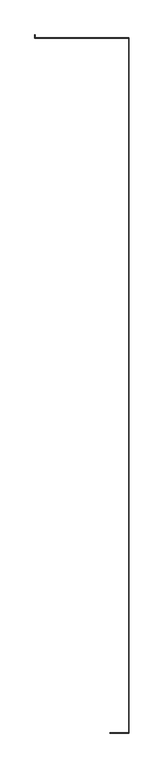
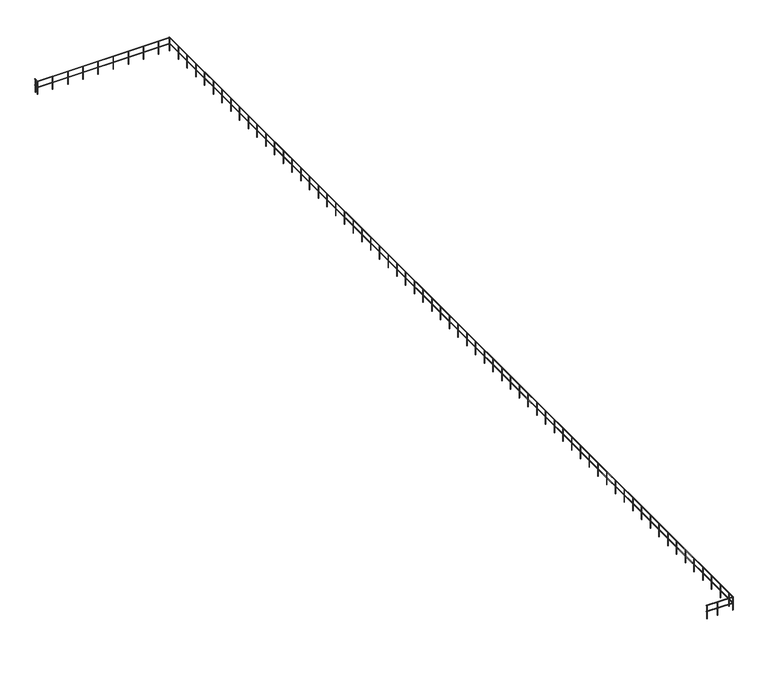
"""IFC4 building model written with IfcOpenShell, lengths in millimetres: railing geometry."""

from ifc_helpers import new_model, si_unit, point, frame, frame_2d, origin, place, context, project, spatial, circle_curve, ellipse_curve, trimmed, segment, composite_curve, outline, extrude, source, transform, mapped, element, save
from ifc_brep_helpers import plane_surface, cylinder_surface, advanced_brep


def railing_6406d98e(model_context):
    return source(origin(), model_context, "Body", "SolidModel", [
        advanced_brep(
        [(65806.3017909, 71787.4208589, 885.0), (65776.3017909, 71787.4208589, 885.0), (65806.3017909, 71467.0208589, 885.0), (65776.3017909, 71437.0208589, 885.0), (76281.0, 71467.0208589, 885.0), (76251.0, 71437.0208589, 885.0), (76281.0, -5867.9791411, 885.0), (76251.0, -5837.9791411, 885.0), (74181.0, -5867.9791411, 885.0), (74181.0, -5837.9791411, 885.0)],
        [
            (0, 1, circle_curve(frame((65791.3017909, 71787.4208589, 885.0), z_axis=(0.0, 1.0, 0.0), x_axis=(-1.0, 0.0, 0.0)), 15.0)),
            (1, 0, circle_curve(frame((65791.3017909, 71787.4208589, 885.0), z_axis=(0.0, 1.0, 0.0), x_axis=(-1.0, 0.0, 0.0)), 15.0)),
            (0, 2),
            (2, 3, ellipse_curve(frame((65791.3017909, 71452.0208589, 885.0), z_axis=(-0.7071067811865464, 0.7071067811865487, 0.0), x_axis=(0.7071067811865487, 0.7071067811865464, 0.0)), 21.2132034, 15.0)),
            (3, 1),
            (3, 2, ellipse_curve(frame((65791.3017909, 71452.0208589, 885.0), z_axis=(-0.7071067811865464, 0.7071067811865487, 0.0), x_axis=(0.7071067811865487, 0.7071067811865464, 0.0)), 21.2132034, 15.0)),
            (2, 4),
            (4, 5, ellipse_curve(frame((76266.0, 71452.0208589, 885.0), z_axis=(-0.7071067811865458, 0.7071067811865492, 0.0), x_axis=(-0.7071067811865492, -0.7071067811865458, 0.0)), 21.2132034, 15.0)),
            (5, 3),
            (5, 4, ellipse_curve(frame((76266.0, 71452.0208589, 885.0), z_axis=(-0.7071067811865458, 0.7071067811865492, 0.0), x_axis=(-0.7071067811865492, -0.7071067811865458, 0.0)), 21.2132034, 15.0)),
            (4, 6),
            (6, 7, ellipse_curve(frame((76266.0, -5852.9791411, 885.0), z_axis=(0.7071067811865491, 0.7071067811865458, 0.0), x_axis=(-0.7071067811865457, 0.7071067811865493, 0.0)), 21.2132034, 15.0)),
            (7, 5),
            (7, 6, ellipse_curve(frame((76266.0, -5852.9791411, 885.0), z_axis=(0.7071067811865491, 0.7071067811865458, 0.0), x_axis=(-0.7071067811865457, 0.7071067811865493, 0.0)), 21.2132034, 15.0)),
            (8, 9, circle_curve(frame((74181.0, -5852.9791411, 885.0), z_axis=(-1.0, 0.0, 0.0), x_axis=(0.0, 1.0, 0.0)), 15.0)),
            (9, 8, circle_curve(frame((74181.0, -5852.9791411, 885.0), z_axis=(-1.0, 0.0, 0.0), x_axis=(0.0, 1.0, 0.0)), 15.0)),
            (6, 8),
            (9, 7),
        ],
        [
            plane_surface(frame((65791.3017909, 71787.4208589, 900.0), z_axis=(0.0, 1.0, 0.0), x_axis=(0.0, 0.0, -1.0))),
            cylinder_surface(frame((65791.3017909, 71787.4208589, 885.0), z_axis=(0.0, 1.0, 0.0), x_axis=(-1.0, 0.0, 0.0)), 15.0),
            cylinder_surface(frame((65791.3017909, 71452.0208589, 885.0), z_axis=(-1.0, 0.0, 0.0), x_axis=(0.0, -1.0, 0.0)), 15.0),
            cylinder_surface(frame((76266.0, 71452.0208589, 885.0), z_axis=(0.0, 1.0, 0.0), x_axis=(-1.0, 0.0, 0.0)), 15.0),
            plane_surface(frame((74181.0, -5852.9791411, 900.0), z_axis=(-1.0, 0.0, 0.0), x_axis=(0.0, -1.0, 0.0))),
            cylinder_surface(frame((76266.0, -5852.9791411, 885.0), z_axis=(1.0, 0.0, 0.0), x_axis=(0.0, 1.0, 0.0)), 15.0),
        ],
        [
            (0, [[1, 2]]),
            (1, [[-1, 3, 4, 5]]),
            (1, [[-2, -5, 6, -3]]),
            (2, [[-4, 7, 8, 9]]),
            (2, [[-6, -9, 10, -7]]),
            (3, [[-8, 11, 12, 13]]),
            (3, [[-10, -13, 14, -11]]),
            (4, [[15, 16]]),
            (5, [[-12, 17, -16, 18]]),
            (5, [[-14, -18, -15, -17]]),
        ],
    ),
        advanced_brep(
        [(65806.3017909, 71787.4208589, 1385.0), (65776.3017909, 71787.4208589, 1385.0), (65806.3017909, 71467.0208589, 1385.0), (65776.3017909, 71437.0208589, 1385.0), (76281.0, 71467.0208589, 1385.0), (76251.0, 71437.0208589, 1385.0), (76281.0, -5867.9791411, 1385.0), (76251.0, -5837.9791411, 1385.0), (74181.0, -5867.9791411, 1385.0), (74181.0, -5837.9791411, 1385.0)],
        [
            (0, 1, circle_curve(frame((65791.3017909, 71787.4208589, 1385.0), z_axis=(0.0, 1.0, 0.0), x_axis=(-1.0, 0.0, 0.0)), 15.0)),
            (1, 0, circle_curve(frame((65791.3017909, 71787.4208589, 1385.0), z_axis=(0.0, 1.0, 0.0), x_axis=(-1.0, 0.0, 0.0)), 15.0)),
            (0, 2),
            (2, 3, ellipse_curve(frame((65791.3017909, 71452.0208589, 1385.0), z_axis=(-0.7071067811865464, 0.7071067811865487, 0.0), x_axis=(0.7071067811865487, 0.7071067811865464, 0.0)), 21.2132034, 15.0)),
            (3, 1),
            (3, 2, ellipse_curve(frame((65791.3017909, 71452.0208589, 1385.0), z_axis=(-0.7071067811865464, 0.7071067811865487, 0.0), x_axis=(0.7071067811865487, 0.7071067811865464, 0.0)), 21.2132034, 15.0)),
            (2, 4),
            (4, 5, ellipse_curve(frame((76266.0, 71452.0208589, 1385.0), z_axis=(-0.7071067811865458, 0.7071067811865492, 0.0), x_axis=(-0.7071067811865492, -0.7071067811865458, 0.0)), 21.2132034, 15.0)),
            (5, 3),
            (5, 4, ellipse_curve(frame((76266.0, 71452.0208589, 1385.0), z_axis=(-0.7071067811865458, 0.7071067811865492, 0.0), x_axis=(-0.7071067811865492, -0.7071067811865458, 0.0)), 21.2132034, 15.0)),
            (4, 6),
            (6, 7, ellipse_curve(frame((76266.0, -5852.9791411, 1385.0), z_axis=(0.7071067811865491, 0.7071067811865458, 0.0), x_axis=(-0.7071067811865457, 0.7071067811865493, 0.0)), 21.2132034, 15.0)),
            (7, 5),
            (7, 6, ellipse_curve(frame((76266.0, -5852.9791411, 1385.0), z_axis=(0.7071067811865491, 0.7071067811865458, 0.0), x_axis=(-0.7071067811865457, 0.7071067811865493, 0.0)), 21.2132034, 15.0)),
            (8, 9, circle_curve(frame((74181.0, -5852.9791411, 1385.0), z_axis=(-1.0, 0.0, 0.0), x_axis=(0.0, 1.0, 0.0)), 15.0)),
            (9, 8, circle_curve(frame((74181.0, -5852.9791411, 1385.0), z_axis=(-1.0, 0.0, 0.0), x_axis=(0.0, 1.0, 0.0)), 15.0)),
            (6, 8),
            (9, 7),
        ],
        [
            plane_surface(frame((65791.3017909, 71787.4208589, 1400.0), z_axis=(0.0, 1.0, 0.0), x_axis=(0.0, 0.0, -1.0))),
            cylinder_surface(frame((65791.3017909, 71787.4208589, 1385.0), z_axis=(0.0, 1.0, 0.0), x_axis=(-1.0, 0.0, 0.0)), 15.0),
            cylinder_surface(frame((65791.3017909, 71452.0208589, 1385.0), z_axis=(-1.0, 0.0, 0.0), x_axis=(0.0, -1.0, 0.0)), 15.0),
            cylinder_surface(frame((76266.0, 71452.0208589, 1385.0), z_axis=(0.0, 1.0, 0.0), x_axis=(-1.0, 0.0, 0.0)), 15.0),
            plane_surface(frame((74181.0, -5852.9791411, 1400.0), z_axis=(-1.0, 0.0, 0.0), x_axis=(0.0, -1.0, 0.0))),
            cylinder_surface(frame((76266.0, -5852.9791411, 1385.0), z_axis=(1.0, 0.0, 0.0), x_axis=(0.0, 1.0, 0.0)), 15.0),
        ],
        [
            (0, [[1, 2]]),
            (1, [[-1, 3, 4, 5]]),
            (1, [[-2, -5, 6, -3]]),
            (2, [[-4, 7, 8, 9]]),
            (2, [[-6, -9, 10, -7]]),
            (3, [[-8, 11, 12, 13]]),
            (3, [[-10, -13, 14, -11]]),
            (4, [[15, 16]]),
            (5, [[-12, 17, -16, 18]]),
            (5, [[-14, -18, -15, -17]]),
        ],
    ),
        extrude(outline(composite_curve([segment(trimmed(circle_curve(frame_2d((75066.0, -5852.9791411)), 15.0), [point((75066.0, -5867.9791411))], [point((75066.0, -5837.9791411))], False, "CARTESIAN"), True, "CONTINUOUS"), segment(trimmed(circle_curve(frame_2d((75066.0, -5852.9791411)), 15.0), [point((75066.0, -5837.9791411))], [point((75066.0, -5867.9791411))], False, "CARTESIAN"), True, "CONTINUOUS")], self_intersect=False)), frame((0.0, 0.0, 300.0), z_axis=(0.0, 0.0, 1.0), x_axis=(1.0, 0.0, 0.0)), (0.0, 0.0, 1.0), 1070.0),
        extrude(outline(composite_curve([segment(trimmed(circle_curve(frame_2d((76266.0, -5347.9791411)), 15.0), [point((76281.0, -5347.9791411))], [point((76251.0, -5347.9791411))], False, "CARTESIAN"), True, "CONTINUOUS"), segment(trimmed(circle_curve(frame_2d((76266.0, -5347.9791411)), 15.0), [point((76251.0, -5347.9791411))], [point((76281.0, -5347.9791411))], False, "CARTESIAN"), True, "CONTINUOUS")], self_intersect=False)), frame((0.0, 0.0, 300.0), z_axis=(0.0, 0.0, 1.0), x_axis=(1.0, 0.0, 0.0)), (0.0, 0.0, 1.0), 1070.0),
        extrude(outline(composite_curve([segment(trimmed(circle_curve(frame_2d((76266.0, -4147.9791411)), 15.0), [point((76281.0, -4147.9791411))], [point((76251.0, -4147.9791411))], False, "CARTESIAN"), True, "CONTINUOUS"), segment(trimmed(circle_curve(frame_2d((76266.0, -4147.9791411)), 15.0), [point((76251.0, -4147.9791411))], [point((76281.0, -4147.9791411))], False, "CARTESIAN"), True, "CONTINUOUS")], self_intersect=False)), frame((0.0, 0.0, 300.0), z_axis=(0.0, 0.0, 1.0), x_axis=(1.0, 0.0, 0.0)), (0.0, 0.0, 1.0), 1070.0),
        extrude(outline(composite_curve([segment(trimmed(circle_curve(frame_2d((76266.0, -2947.9791411)), 15.0), [point((76281.0, -2947.9791411))], [point((76251.0, -2947.9791411))], False, "CARTESIAN"), True, "CONTINUOUS"), segment(trimmed(circle_curve(frame_2d((76266.0, -2947.9791411)), 15.0), [point((76251.0, -2947.9791411))], [point((76281.0, -2947.9791411))], False, "CARTESIAN"), True, "CONTINUOUS")], self_intersect=False)), frame((0.0, 0.0, 300.0), z_axis=(0.0, 0.0, 1.0), x_axis=(1.0, 0.0, 0.0)), (0.0, 0.0, 1.0), 1070.0),
        extrude(outline(composite_curve([segment(trimmed(circle_curve(frame_2d((76266.0, -1747.9791411)), 15.0), [point((76281.0, -1747.9791411))], [point((76251.0, -1747.9791411))], False, "CARTESIAN"), True, "CONTINUOUS"), segment(trimmed(circle_curve(frame_2d((76266.0, -1747.9791411)), 15.0), [point((76251.0, -1747.9791411))], [point((76281.0, -1747.9791411))], False, "CARTESIAN"), True, "CONTINUOUS")], self_intersect=False)), frame((0.0, 0.0, 300.0), z_axis=(0.0, 0.0, 1.0), x_axis=(1.0, 0.0, 0.0)), (0.0, 0.0, 1.0), 1070.0),
        extrude(outline(composite_curve([segment(trimmed(circle_curve(frame_2d((76266.0, -547.9791411)), 15.0), [point((76281.0, -547.9791411))], [point((76251.0, -547.9791411))], False, "CARTESIAN"), True, "CONTINUOUS"), segment(trimmed(circle_curve(frame_2d((76266.0, -547.9791411)), 15.0), [point((76251.0, -547.9791411))], [point((76281.0, -547.9791411))], False, "CARTESIAN"), True, "CONTINUOUS")], self_intersect=False)), frame((0.0, 0.0, 300.0), z_axis=(0.0, 0.0, 1.0), x_axis=(1.0, 0.0, 0.0)), (0.0, 0.0, 1.0), 1070.0),
        extrude(outline(composite_curve([segment(trimmed(circle_curve(frame_2d((76266.0, 652.0208589)), 15.0), [point((76281.0, 652.0208589))], [point((76251.0, 652.0208589))], False, "CARTESIAN"), True, "CONTINUOUS"), segment(trimmed(circle_curve(frame_2d((76266.0, 652.0208589)), 15.0), [point((76251.0, 652.0208589))], [point((76281.0, 652.0208589))], False, "CARTESIAN"), True, "CONTINUOUS")], self_intersect=False)), frame((0.0, 0.0, 300.0), z_axis=(0.0, 0.0, 1.0), x_axis=(1.0, 0.0, 0.0)), (0.0, 0.0, 1.0), 1070.0),
        extrude(outline(composite_curve([segment(trimmed(circle_curve(frame_2d((76266.0, 1852.0208589)), 15.0), [point((76281.0, 1852.0208589))], [point((76251.0, 1852.0208589))], False, "CARTESIAN"), True, "CONTINUOUS"), segment(trimmed(circle_curve(frame_2d((76266.0, 1852.0208589)), 15.0), [point((76251.0, 1852.0208589))], [point((76281.0, 1852.0208589))], False, "CARTESIAN"), True, "CONTINUOUS")], self_intersect=False)), frame((0.0, 0.0, 300.0), z_axis=(0.0, 0.0, 1.0), x_axis=(1.0, 0.0, 0.0)), (0.0, 0.0, 1.0), 1070.0),
        extrude(outline(composite_curve([segment(trimmed(circle_curve(frame_2d((76266.0, 3052.0208589)), 15.0), [point((76281.0, 3052.0208589))], [point((76251.0, 3052.0208589))], False, "CARTESIAN"), True, "CONTINUOUS"), segment(trimmed(circle_curve(frame_2d((76266.0, 3052.0208589)), 15.0), [point((76251.0, 3052.0208589))], [point((76281.0, 3052.0208589))], False, "CARTESIAN"), True, "CONTINUOUS")], self_intersect=False)), frame((0.0, 0.0, 300.0), z_axis=(0.0, 0.0, 1.0), x_axis=(1.0, 0.0, 0.0)), (0.0, 0.0, 1.0), 1070.0),
        extrude(outline(composite_curve([segment(trimmed(circle_curve(frame_2d((76266.0, 4252.0208589)), 15.0), [point((76281.0, 4252.0208589))], [point((76251.0, 4252.0208589))], False, "CARTESIAN"), True, "CONTINUOUS"), segment(trimmed(circle_curve(frame_2d((76266.0, 4252.0208589)), 15.0), [point((76251.0, 4252.0208589))], [point((76281.0, 4252.0208589))], False, "CARTESIAN"), True, "CONTINUOUS")], self_intersect=False)), frame((0.0, 0.0, 300.0), z_axis=(0.0, 0.0, 1.0), x_axis=(1.0, 0.0, 0.0)), (0.0, 0.0, 1.0), 1070.0),
        extrude(outline(composite_curve([segment(trimmed(circle_curve(frame_2d((76266.0, 5452.0208589)), 15.0), [point((76281.0, 5452.0208589))], [point((76251.0, 5452.0208589))], False, "CARTESIAN"), True, "CONTINUOUS"), segment(trimmed(circle_curve(frame_2d((76266.0, 5452.0208589)), 15.0), [point((76251.0, 5452.0208589))], [point((76281.0, 5452.0208589))], False, "CARTESIAN"), True, "CONTINUOUS")], self_intersect=False)), frame((0.0, 0.0, 300.0), z_axis=(0.0, 0.0, 1.0), x_axis=(1.0, 0.0, 0.0)), (0.0, 0.0, 1.0), 1070.0),
        extrude(outline(composite_curve([segment(trimmed(circle_curve(frame_2d((76266.0, 6652.0208589)), 15.0), [point((76281.0, 6652.0208589))], [point((76251.0, 6652.0208589))], False, "CARTESIAN"), True, "CONTINUOUS"), segment(trimmed(circle_curve(frame_2d((76266.0, 6652.0208589)), 15.0), [point((76251.0, 6652.0208589))], [point((76281.0, 6652.0208589))], False, "CARTESIAN"), True, "CONTINUOUS")], self_intersect=False)), frame((0.0, 0.0, 300.0), z_axis=(0.0, 0.0, 1.0), x_axis=(1.0, 0.0, 0.0)), (0.0, 0.0, 1.0), 1070.0),
        extrude(outline(composite_curve([segment(trimmed(circle_curve(frame_2d((76266.0, 7852.0208589)), 15.0), [point((76281.0, 7852.0208589))], [point((76251.0, 7852.0208589))], False, "CARTESIAN"), True, "CONTINUOUS"), segment(trimmed(circle_curve(frame_2d((76266.0, 7852.0208589)), 15.0), [point((76251.0, 7852.0208589))], [point((76281.0, 7852.0208589))], False, "CARTESIAN"), True, "CONTINUOUS")], self_intersect=False)), frame((0.0, 0.0, 300.0), z_axis=(0.0, 0.0, 1.0), x_axis=(1.0, 0.0, 0.0)), (0.0, 0.0, 1.0), 1070.0),
        extrude(outline(composite_curve([segment(trimmed(circle_curve(frame_2d((76266.0, 9052.0208589)), 15.0), [point((76281.0, 9052.0208589))], [point((76251.0, 9052.0208589))], False, "CARTESIAN"), True, "CONTINUOUS"), segment(trimmed(circle_curve(frame_2d((76266.0, 9052.0208589)), 15.0), [point((76251.0, 9052.0208589))], [point((76281.0, 9052.0208589))], False, "CARTESIAN"), True, "CONTINUOUS")], self_intersect=False)), frame((0.0, 0.0, 300.0), z_axis=(0.0, 0.0, 1.0), x_axis=(1.0, 0.0, 0.0)), (0.0, 0.0, 1.0), 1070.0),
        extrude(outline(composite_curve([segment(trimmed(circle_curve(frame_2d((76266.0, 10252.0208589)), 15.0), [point((76281.0, 10252.0208589))], [point((76251.0, 10252.0208589))], False, "CARTESIAN"), True, "CONTINUOUS"), segment(trimmed(circle_curve(frame_2d((76266.0, 10252.0208589)), 15.0), [point((76251.0, 10252.0208589))], [point((76281.0, 10252.0208589))], False, "CARTESIAN"), True, "CONTINUOUS")], self_intersect=False)), frame((0.0, 0.0, 300.0), z_axis=(0.0, 0.0, 1.0), x_axis=(1.0, 0.0, 0.0)), (0.0, 0.0, 1.0), 1070.0),
        extrude(outline(composite_curve([segment(trimmed(circle_curve(frame_2d((76266.0, 11452.0208589)), 15.0), [point((76281.0, 11452.0208589))], [point((76251.0, 11452.0208589))], False, "CARTESIAN"), True, "CONTINUOUS"), segment(trimmed(circle_curve(frame_2d((76266.0, 11452.0208589)), 15.0), [point((76251.0, 11452.0208589))], [point((76281.0, 11452.0208589))], False, "CARTESIAN"), True, "CONTINUOUS")], self_intersect=False)), frame((0.0, 0.0, 300.0), z_axis=(0.0, 0.0, 1.0), x_axis=(1.0, 0.0, 0.0)), (0.0, 0.0, 1.0), 1070.0),
        extrude(outline(composite_curve([segment(trimmed(circle_curve(frame_2d((76266.0, 12652.0208589)), 15.0), [point((76281.0, 12652.0208589))], [point((76251.0, 12652.0208589))], False, "CARTESIAN"), True, "CONTINUOUS"), segment(trimmed(circle_curve(frame_2d((76266.0, 12652.0208589)), 15.0), [point((76251.0, 12652.0208589))], [point((76281.0, 12652.0208589))], False, "CARTESIAN"), True, "CONTINUOUS")], self_intersect=False)), frame((0.0, 0.0, 300.0), z_axis=(0.0, 0.0, 1.0), x_axis=(1.0, 0.0, 0.0)), (0.0, 0.0, 1.0), 1070.0),
        extrude(outline(composite_curve([segment(trimmed(circle_curve(frame_2d((76266.0, 13852.0208589)), 15.0), [point((76281.0, 13852.0208589))], [point((76251.0, 13852.0208589))], False, "CARTESIAN"), True, "CONTINUOUS"), segment(trimmed(circle_curve(frame_2d((76266.0, 13852.0208589)), 15.0), [point((76251.0, 13852.0208589))], [point((76281.0, 13852.0208589))], False, "CARTESIAN"), True, "CONTINUOUS")], self_intersect=False)), frame((0.0, 0.0, 300.0), z_axis=(0.0, 0.0, 1.0), x_axis=(1.0, 0.0, 0.0)), (0.0, 0.0, 1.0), 1070.0),
        extrude(outline(composite_curve([segment(trimmed(circle_curve(frame_2d((76266.0, 15052.0208589)), 15.0), [point((76281.0, 15052.0208589))], [point((76251.0, 15052.0208589))], False, "CARTESIAN"), True, "CONTINUOUS"), segment(trimmed(circle_curve(frame_2d((76266.0, 15052.0208589)), 15.0), [point((76251.0, 15052.0208589))], [point((76281.0, 15052.0208589))], False, "CARTESIAN"), True, "CONTINUOUS")], self_intersect=False)), frame((0.0, 0.0, 300.0), z_axis=(0.0, 0.0, 1.0), x_axis=(1.0, 0.0, 0.0)), (0.0, 0.0, 1.0), 1070.0),
        extrude(outline(composite_curve([segment(trimmed(circle_curve(frame_2d((76266.0, 16252.0208589)), 15.0), [point((76281.0, 16252.0208589))], [point((76251.0, 16252.0208589))], False, "CARTESIAN"), True, "CONTINUOUS"), segment(trimmed(circle_curve(frame_2d((76266.0, 16252.0208589)), 15.0), [point((76251.0, 16252.0208589))], [point((76281.0, 16252.0208589))], False, "CARTESIAN"), True, "CONTINUOUS")], self_intersect=False)), frame((0.0, 0.0, 300.0), z_axis=(0.0, 0.0, 1.0), x_axis=(1.0, 0.0, 0.0)), (0.0, 0.0, 1.0), 1070.0),
        extrude(outline(composite_curve([segment(trimmed(circle_curve(frame_2d((76266.0, 17452.0208589)), 15.0), [point((76281.0, 17452.0208589))], [point((76251.0, 17452.0208589))], False, "CARTESIAN"), True, "CONTINUOUS"), segment(trimmed(circle_curve(frame_2d((76266.0, 17452.0208589)), 15.0), [point((76251.0, 17452.0208589))], [point((76281.0, 17452.0208589))], False, "CARTESIAN"), True, "CONTINUOUS")], self_intersect=False)), frame((0.0, 0.0, 300.0), z_axis=(0.0, 0.0, 1.0), x_axis=(1.0, 0.0, 0.0)), (0.0, 0.0, 1.0), 1070.0),
        extrude(outline(composite_curve([segment(trimmed(circle_curve(frame_2d((76266.0, 18652.0208589)), 15.0), [point((76281.0, 18652.0208589))], [point((76251.0, 18652.0208589))], False, "CARTESIAN"), True, "CONTINUOUS"), segment(trimmed(circle_curve(frame_2d((76266.0, 18652.0208589)), 15.0), [point((76251.0, 18652.0208589))], [point((76281.0, 18652.0208589))], False, "CARTESIAN"), True, "CONTINUOUS")], self_intersect=False)), frame((0.0, 0.0, 300.0), z_axis=(0.0, 0.0, 1.0), x_axis=(1.0, 0.0, 0.0)), (0.0, 0.0, 1.0), 1070.0),
        extrude(outline(composite_curve([segment(trimmed(circle_curve(frame_2d((76266.0, 19852.0208589)), 15.0), [point((76281.0, 19852.0208589))], [point((76251.0, 19852.0208589))], False, "CARTESIAN"), True, "CONTINUOUS"), segment(trimmed(circle_curve(frame_2d((76266.0, 19852.0208589)), 15.0), [point((76251.0, 19852.0208589))], [point((76281.0, 19852.0208589))], False, "CARTESIAN"), True, "CONTINUOUS")], self_intersect=False)), frame((0.0, 0.0, 300.0), z_axis=(0.0, 0.0, 1.0), x_axis=(1.0, 0.0, 0.0)), (0.0, 0.0, 1.0), 1070.0),
        extrude(outline(composite_curve([segment(trimmed(circle_curve(frame_2d((76266.0, 21052.0208589)), 15.0), [point((76281.0, 21052.0208589))], [point((76251.0, 21052.0208589))], False, "CARTESIAN"), True, "CONTINUOUS"), segment(trimmed(circle_curve(frame_2d((76266.0, 21052.0208589)), 15.0), [point((76251.0, 21052.0208589))], [point((76281.0, 21052.0208589))], False, "CARTESIAN"), True, "CONTINUOUS")], self_intersect=False)), frame((0.0, 0.0, 300.0), z_axis=(0.0, 0.0, 1.0), x_axis=(1.0, 0.0, 0.0)), (0.0, 0.0, 1.0), 1070.0),
        extrude(outline(composite_curve([segment(trimmed(circle_curve(frame_2d((76266.0, 22252.0208589)), 15.0), [point((76281.0, 22252.0208589))], [point((76251.0, 22252.0208589))], False, "CARTESIAN"), True, "CONTINUOUS"), segment(trimmed(circle_curve(frame_2d((76266.0, 22252.0208589)), 15.0), [point((76251.0, 22252.0208589))], [point((76281.0, 22252.0208589))], False, "CARTESIAN"), True, "CONTINUOUS")], self_intersect=False)), frame((0.0, 0.0, 300.0), z_axis=(0.0, 0.0, 1.0), x_axis=(1.0, 0.0, 0.0)), (0.0, 0.0, 1.0), 1070.0),
        extrude(outline(composite_curve([segment(trimmed(circle_curve(frame_2d((76266.0, 23452.0208589)), 15.0), [point((76281.0, 23452.0208589))], [point((76251.0, 23452.0208589))], False, "CARTESIAN"), True, "CONTINUOUS"), segment(trimmed(circle_curve(frame_2d((76266.0, 23452.0208589)), 15.0), [point((76251.0, 23452.0208589))], [point((76281.0, 23452.0208589))], False, "CARTESIAN"), True, "CONTINUOUS")], self_intersect=False)), frame((0.0, 0.0, 300.0), z_axis=(0.0, 0.0, 1.0), x_axis=(1.0, 0.0, 0.0)), (0.0, 0.0, 1.0), 1070.0),
        extrude(outline(composite_curve([segment(trimmed(circle_curve(frame_2d((76266.0, 24652.0208589)), 15.0), [point((76281.0, 24652.0208589))], [point((76251.0, 24652.0208589))], False, "CARTESIAN"), True, "CONTINUOUS"), segment(trimmed(circle_curve(frame_2d((76266.0, 24652.0208589)), 15.0), [point((76251.0, 24652.0208589))], [point((76281.0, 24652.0208589))], False, "CARTESIAN"), True, "CONTINUOUS")], self_intersect=False)), frame((0.0, 0.0, 300.0), z_axis=(0.0, 0.0, 1.0), x_axis=(1.0, 0.0, 0.0)), (0.0, 0.0, 1.0), 1070.0),
        extrude(outline(composite_curve([segment(trimmed(circle_curve(frame_2d((76266.0, 25852.0208589)), 15.0), [point((76281.0, 25852.0208589))], [point((76251.0, 25852.0208589))], False, "CARTESIAN"), True, "CONTINUOUS"), segment(trimmed(circle_curve(frame_2d((76266.0, 25852.0208589)), 15.0), [point((76251.0, 25852.0208589))], [point((76281.0, 25852.0208589))], False, "CARTESIAN"), True, "CONTINUOUS")], self_intersect=False)), frame((0.0, 0.0, 300.0), z_axis=(0.0, 0.0, 1.0), x_axis=(1.0, 0.0, 0.0)), (0.0, 0.0, 1.0), 1070.0),
        extrude(outline(composite_curve([segment(trimmed(circle_curve(frame_2d((76266.0, 27052.0208589)), 15.0), [point((76281.0, 27052.0208589))], [point((76251.0, 27052.0208589))], False, "CARTESIAN"), True, "CONTINUOUS"), segment(trimmed(circle_curve(frame_2d((76266.0, 27052.0208589)), 15.0), [point((76251.0, 27052.0208589))], [point((76281.0, 27052.0208589))], False, "CARTESIAN"), True, "CONTINUOUS")], self_intersect=False)), frame((0.0, 0.0, 300.0), z_axis=(0.0, 0.0, 1.0), x_axis=(1.0, 0.0, 0.0)), (0.0, 0.0, 1.0), 1070.0),
        extrude(outline(composite_curve([segment(trimmed(circle_curve(frame_2d((76266.0, 28252.0208589)), 15.0), [point((76281.0, 28252.0208589))], [point((76251.0, 28252.0208589))], False, "CARTESIAN"), True, "CONTINUOUS"), segment(trimmed(circle_curve(frame_2d((76266.0, 28252.0208589)), 15.0), [point((76251.0, 28252.0208589))], [point((76281.0, 28252.0208589))], False, "CARTESIAN"), True, "CONTINUOUS")], self_intersect=False)), frame((0.0, 0.0, 300.0), z_axis=(0.0, 0.0, 1.0), x_axis=(1.0, 0.0, 0.0)), (0.0, 0.0, 1.0), 1070.0),
        extrude(outline(composite_curve([segment(trimmed(circle_curve(frame_2d((76266.0, 29452.0208589)), 15.0), [point((76281.0, 29452.0208589))], [point((76251.0, 29452.0208589))], False, "CARTESIAN"), True, "CONTINUOUS"), segment(trimmed(circle_curve(frame_2d((76266.0, 29452.0208589)), 15.0), [point((76251.0, 29452.0208589))], [point((76281.0, 29452.0208589))], False, "CARTESIAN"), True, "CONTINUOUS")], self_intersect=False)), frame((0.0, 0.0, 300.0), z_axis=(0.0, 0.0, 1.0), x_axis=(1.0, 0.0, 0.0)), (0.0, 0.0, 1.0), 1070.0),
        extrude(outline(composite_curve([segment(trimmed(circle_curve(frame_2d((76266.0, 30652.0208589)), 15.0), [point((76281.0, 30652.0208589))], [point((76251.0, 30652.0208589))], False, "CARTESIAN"), True, "CONTINUOUS"), segment(trimmed(circle_curve(frame_2d((76266.0, 30652.0208589)), 15.0), [point((76251.0, 30652.0208589))], [point((76281.0, 30652.0208589))], False, "CARTESIAN"), True, "CONTINUOUS")], self_intersect=False)), frame((0.0, 0.0, 300.0), z_axis=(0.0, 0.0, 1.0), x_axis=(1.0, 0.0, 0.0)), (0.0, 0.0, 1.0), 1070.0),
        extrude(outline(composite_curve([segment(trimmed(circle_curve(frame_2d((76266.0, 31852.0208589)), 15.0), [point((76281.0, 31852.0208589))], [point((76251.0, 31852.0208589))], False, "CARTESIAN"), True, "CONTINUOUS"), segment(trimmed(circle_curve(frame_2d((76266.0, 31852.0208589)), 15.0), [point((76251.0, 31852.0208589))], [point((76281.0, 31852.0208589))], False, "CARTESIAN"), True, "CONTINUOUS")], self_intersect=False)), frame((0.0, 0.0, 300.0), z_axis=(0.0, 0.0, 1.0), x_axis=(1.0, 0.0, 0.0)), (0.0, 0.0, 1.0), 1070.0),
        extrude(outline(composite_curve([segment(trimmed(circle_curve(frame_2d((76266.0, 33052.0208589)), 15.0), [point((76281.0, 33052.0208589))], [point((76251.0, 33052.0208589))], False, "CARTESIAN"), True, "CONTINUOUS"), segment(trimmed(circle_curve(frame_2d((76266.0, 33052.0208589)), 15.0), [point((76251.0, 33052.0208589))], [point((76281.0, 33052.0208589))], False, "CARTESIAN"), True, "CONTINUOUS")], self_intersect=False)), frame((0.0, 0.0, 300.0), z_axis=(0.0, 0.0, 1.0), x_axis=(1.0, 0.0, 0.0)), (0.0, 0.0, 1.0), 1070.0),
        extrude(outline(composite_curve([segment(trimmed(circle_curve(frame_2d((76266.0, 34252.0208589)), 15.0), [point((76281.0, 34252.0208589))], [point((76251.0, 34252.0208589))], False, "CARTESIAN"), True, "CONTINUOUS"), segment(trimmed(circle_curve(frame_2d((76266.0, 34252.0208589)), 15.0), [point((76251.0, 34252.0208589))], [point((76281.0, 34252.0208589))], False, "CARTESIAN"), True, "CONTINUOUS")], self_intersect=False)), frame((0.0, 0.0, 300.0), z_axis=(0.0, 0.0, 1.0), x_axis=(1.0, 0.0, 0.0)), (0.0, 0.0, 1.0), 1070.0),
        extrude(outline(composite_curve([segment(trimmed(circle_curve(frame_2d((76266.0, 35452.0208589)), 15.0), [point((76281.0, 35452.0208589))], [point((76251.0, 35452.0208589))], False, "CARTESIAN"), True, "CONTINUOUS"), segment(trimmed(circle_curve(frame_2d((76266.0, 35452.0208589)), 15.0), [point((76251.0, 35452.0208589))], [point((76281.0, 35452.0208589))], False, "CARTESIAN"), True, "CONTINUOUS")], self_intersect=False)), frame((0.0, 0.0, 300.0), z_axis=(0.0, 0.0, 1.0), x_axis=(1.0, 0.0, 0.0)), (0.0, 0.0, 1.0), 1070.0),
        extrude(outline(composite_curve([segment(trimmed(circle_curve(frame_2d((76266.0, 36652.0208589)), 15.0), [point((76281.0, 36652.0208589))], [point((76251.0, 36652.0208589))], False, "CARTESIAN"), True, "CONTINUOUS"), segment(trimmed(circle_curve(frame_2d((76266.0, 36652.0208589)), 15.0), [point((76251.0, 36652.0208589))], [point((76281.0, 36652.0208589))], False, "CARTESIAN"), True, "CONTINUOUS")], self_intersect=False)), frame((0.0, 0.0, 300.0), z_axis=(0.0, 0.0, 1.0), x_axis=(1.0, 0.0, 0.0)), (0.0, 0.0, 1.0), 1070.0),
        extrude(outline(composite_curve([segment(trimmed(circle_curve(frame_2d((76266.0, 37852.0208589)), 15.0), [point((76281.0, 37852.0208589))], [point((76251.0, 37852.0208589))], False, "CARTESIAN"), True, "CONTINUOUS"), segment(trimmed(circle_curve(frame_2d((76266.0, 37852.0208589)), 15.0), [point((76251.0, 37852.0208589))], [point((76281.0, 37852.0208589))], False, "CARTESIAN"), True, "CONTINUOUS")], self_intersect=False)), frame((0.0, 0.0, 300.0), z_axis=(0.0, 0.0, 1.0), x_axis=(1.0, 0.0, 0.0)), (0.0, 0.0, 1.0), 1070.0),
        extrude(outline(composite_curve([segment(trimmed(circle_curve(frame_2d((76266.0, 39052.0208589)), 15.0), [point((76281.0, 39052.0208589))], [point((76251.0, 39052.0208589))], False, "CARTESIAN"), True, "CONTINUOUS"), segment(trimmed(circle_curve(frame_2d((76266.0, 39052.0208589)), 15.0), [point((76251.0, 39052.0208589))], [point((76281.0, 39052.0208589))], False, "CARTESIAN"), True, "CONTINUOUS")], self_intersect=False)), frame((0.0, 0.0, 300.0), z_axis=(0.0, 0.0, 1.0), x_axis=(1.0, 0.0, 0.0)), (0.0, 0.0, 1.0), 1070.0),
        extrude(outline(composite_curve([segment(trimmed(circle_curve(frame_2d((76266.0, 40252.0208589)), 15.0), [point((76281.0, 40252.0208589))], [point((76251.0, 40252.0208589))], False, "CARTESIAN"), True, "CONTINUOUS"), segment(trimmed(circle_curve(frame_2d((76266.0, 40252.0208589)), 15.0), [point((76251.0, 40252.0208589))], [point((76281.0, 40252.0208589))], False, "CARTESIAN"), True, "CONTINUOUS")], self_intersect=False)), frame((0.0, 0.0, 300.0), z_axis=(0.0, 0.0, 1.0), x_axis=(1.0, 0.0, 0.0)), (0.0, 0.0, 1.0), 1070.0),
        extrude(outline(composite_curve([segment(trimmed(circle_curve(frame_2d((76266.0, 41452.0208589)), 15.0), [point((76281.0, 41452.0208589))], [point((76251.0, 41452.0208589))], False, "CARTESIAN"), True, "CONTINUOUS"), segment(trimmed(circle_curve(frame_2d((76266.0, 41452.0208589)), 15.0), [point((76251.0, 41452.0208589))], [point((76281.0, 41452.0208589))], False, "CARTESIAN"), True, "CONTINUOUS")], self_intersect=False)), frame((0.0, 0.0, 300.0), z_axis=(0.0, 0.0, 1.0), x_axis=(1.0, 0.0, 0.0)), (0.0, 0.0, 1.0), 1070.0),
        extrude(outline(composite_curve([segment(trimmed(circle_curve(frame_2d((76266.0, 42652.0208589)), 15.0), [point((76281.0, 42652.0208589))], [point((76251.0, 42652.0208589))], False, "CARTESIAN"), True, "CONTINUOUS"), segment(trimmed(circle_curve(frame_2d((76266.0, 42652.0208589)), 15.0), [point((76251.0, 42652.0208589))], [point((76281.0, 42652.0208589))], False, "CARTESIAN"), True, "CONTINUOUS")], self_intersect=False)), frame((0.0, 0.0, 300.0), z_axis=(0.0, 0.0, 1.0), x_axis=(1.0, 0.0, 0.0)), (0.0, 0.0, 1.0), 1070.0),
        extrude(outline(composite_curve([segment(trimmed(circle_curve(frame_2d((76266.0, 43852.0208589)), 15.0), [point((76281.0, 43852.0208589))], [point((76251.0, 43852.0208589))], False, "CARTESIAN"), True, "CONTINUOUS"), segment(trimmed(circle_curve(frame_2d((76266.0, 43852.0208589)), 15.0), [point((76251.0, 43852.0208589))], [point((76281.0, 43852.0208589))], False, "CARTESIAN"), True, "CONTINUOUS")], self_intersect=False)), frame((0.0, 0.0, 300.0), z_axis=(0.0, 0.0, 1.0), x_axis=(1.0, 0.0, 0.0)), (0.0, 0.0, 1.0), 1070.0),
        extrude(outline(composite_curve([segment(trimmed(circle_curve(frame_2d((76266.0, 45052.0208589)), 15.0), [point((76281.0, 45052.0208589))], [point((76251.0, 45052.0208589))], False, "CARTESIAN"), True, "CONTINUOUS"), segment(trimmed(circle_curve(frame_2d((76266.0, 45052.0208589)), 15.0), [point((76251.0, 45052.0208589))], [point((76281.0, 45052.0208589))], False, "CARTESIAN"), True, "CONTINUOUS")], self_intersect=False)), frame((0.0, 0.0, 300.0), z_axis=(0.0, 0.0, 1.0), x_axis=(1.0, 0.0, 0.0)), (0.0, 0.0, 1.0), 1070.0),
        extrude(outline(composite_curve([segment(trimmed(circle_curve(frame_2d((76266.0, 46252.0208589)), 15.0), [point((76281.0, 46252.0208589))], [point((76251.0, 46252.0208589))], False, "CARTESIAN"), True, "CONTINUOUS"), segment(trimmed(circle_curve(frame_2d((76266.0, 46252.0208589)), 15.0), [point((76251.0, 46252.0208589))], [point((76281.0, 46252.0208589))], False, "CARTESIAN"), True, "CONTINUOUS")], self_intersect=False)), frame((0.0, 0.0, 300.0), z_axis=(0.0, 0.0, 1.0), x_axis=(1.0, 0.0, 0.0)), (0.0, 0.0, 1.0), 1070.0),
        extrude(outline(composite_curve([segment(trimmed(circle_curve(frame_2d((76266.0, 47452.0208589)), 15.0), [point((76281.0, 47452.0208589))], [point((76251.0, 47452.0208589))], False, "CARTESIAN"), True, "CONTINUOUS"), segment(trimmed(circle_curve(frame_2d((76266.0, 47452.0208589)), 15.0), [point((76251.0, 47452.0208589))], [point((76281.0, 47452.0208589))], False, "CARTESIAN"), True, "CONTINUOUS")], self_intersect=False)), frame((0.0, 0.0, 300.0), z_axis=(0.0, 0.0, 1.0), x_axis=(1.0, 0.0, 0.0)), (0.0, 0.0, 1.0), 1070.0),
        extrude(outline(composite_curve([segment(trimmed(circle_curve(frame_2d((76266.0, 48652.0208589)), 15.0), [point((76281.0, 48652.0208589))], [point((76251.0, 48652.0208589))], False, "CARTESIAN"), True, "CONTINUOUS"), segment(trimmed(circle_curve(frame_2d((76266.0, 48652.0208589)), 15.0), [point((76251.0, 48652.0208589))], [point((76281.0, 48652.0208589))], False, "CARTESIAN"), True, "CONTINUOUS")], self_intersect=False)), frame((0.0, 0.0, 300.0), z_axis=(0.0, 0.0, 1.0), x_axis=(1.0, 0.0, 0.0)), (0.0, 0.0, 1.0), 1070.0),
        extrude(outline(composite_curve([segment(trimmed(circle_curve(frame_2d((76266.0, 49852.0208589)), 15.0), [point((76281.0, 49852.0208589))], [point((76251.0, 49852.0208589))], False, "CARTESIAN"), True, "CONTINUOUS"), segment(trimmed(circle_curve(frame_2d((76266.0, 49852.0208589)), 15.0), [point((76251.0, 49852.0208589))], [point((76281.0, 49852.0208589))], False, "CARTESIAN"), True, "CONTINUOUS")], self_intersect=False)), frame((0.0, 0.0, 300.0), z_axis=(0.0, 0.0, 1.0), x_axis=(1.0, 0.0, 0.0)), (0.0, 0.0, 1.0), 1070.0),
        extrude(outline(composite_curve([segment(trimmed(circle_curve(frame_2d((76266.0, 51052.0208589)), 15.0), [point((76281.0, 51052.0208589))], [point((76251.0, 51052.0208589))], False, "CARTESIAN"), True, "CONTINUOUS"), segment(trimmed(circle_curve(frame_2d((76266.0, 51052.0208589)), 15.0), [point((76251.0, 51052.0208589))], [point((76281.0, 51052.0208589))], False, "CARTESIAN"), True, "CONTINUOUS")], self_intersect=False)), frame((0.0, 0.0, 300.0), z_axis=(0.0, 0.0, 1.0), x_axis=(1.0, 0.0, 0.0)), (0.0, 0.0, 1.0), 1070.0),
        extrude(outline(composite_curve([segment(trimmed(circle_curve(frame_2d((76266.0, 52252.0208589)), 15.0), [point((76281.0, 52252.0208589))], [point((76251.0, 52252.0208589))], False, "CARTESIAN"), True, "CONTINUOUS"), segment(trimmed(circle_curve(frame_2d((76266.0, 52252.0208589)), 15.0), [point((76251.0, 52252.0208589))], [point((76281.0, 52252.0208589))], False, "CARTESIAN"), True, "CONTINUOUS")], self_intersect=False)), frame((0.0, 0.0, 300.0), z_axis=(0.0, 0.0, 1.0), x_axis=(1.0, 0.0, 0.0)), (0.0, 0.0, 1.0), 1070.0),
        extrude(outline(composite_curve([segment(trimmed(circle_curve(frame_2d((76266.0, 53452.0208589)), 15.0), [point((76281.0, 53452.0208589))], [point((76251.0, 53452.0208589))], False, "CARTESIAN"), True, "CONTINUOUS"), segment(trimmed(circle_curve(frame_2d((76266.0, 53452.0208589)), 15.0), [point((76251.0, 53452.0208589))], [point((76281.0, 53452.0208589))], False, "CARTESIAN"), True, "CONTINUOUS")], self_intersect=False)), frame((0.0, 0.0, 300.0), z_axis=(0.0, 0.0, 1.0), x_axis=(1.0, 0.0, 0.0)), (0.0, 0.0, 1.0), 1070.0),
        extrude(outline(composite_curve([segment(trimmed(circle_curve(frame_2d((76266.0, 54652.0208589)), 15.0), [point((76281.0, 54652.0208589))], [point((76251.0, 54652.0208589))], False, "CARTESIAN"), True, "CONTINUOUS"), segment(trimmed(circle_curve(frame_2d((76266.0, 54652.0208589)), 15.0), [point((76251.0, 54652.0208589))], [point((76281.0, 54652.0208589))], False, "CARTESIAN"), True, "CONTINUOUS")], self_intersect=False)), frame((0.0, 0.0, 300.0), z_axis=(0.0, 0.0, 1.0), x_axis=(1.0, 0.0, 0.0)), (0.0, 0.0, 1.0), 1070.0),
        extrude(outline(composite_curve([segment(trimmed(circle_curve(frame_2d((76266.0, 55852.0208589)), 15.0), [point((76281.0, 55852.0208589))], [point((76251.0, 55852.0208589))], False, "CARTESIAN"), True, "CONTINUOUS"), segment(trimmed(circle_curve(frame_2d((76266.0, 55852.0208589)), 15.0), [point((76251.0, 55852.0208589))], [point((76281.0, 55852.0208589))], False, "CARTESIAN"), True, "CONTINUOUS")], self_intersect=False)), frame((0.0, 0.0, 300.0), z_axis=(0.0, 0.0, 1.0), x_axis=(1.0, 0.0, 0.0)), (0.0, 0.0, 1.0), 1070.0),
        extrude(outline(composite_curve([segment(trimmed(circle_curve(frame_2d((76266.0, 57052.0208589)), 15.0), [point((76281.0, 57052.0208589))], [point((76251.0, 57052.0208589))], False, "CARTESIAN"), True, "CONTINUOUS"), segment(trimmed(circle_curve(frame_2d((76266.0, 57052.0208589)), 15.0), [point((76251.0, 57052.0208589))], [point((76281.0, 57052.0208589))], False, "CARTESIAN"), True, "CONTINUOUS")], self_intersect=False)), frame((0.0, 0.0, 300.0), z_axis=(0.0, 0.0, 1.0), x_axis=(1.0, 0.0, 0.0)), (0.0, 0.0, 1.0), 1070.0),
        extrude(outline(composite_curve([segment(trimmed(circle_curve(frame_2d((76266.0, 58252.0208589)), 15.0), [point((76281.0, 58252.0208589))], [point((76251.0, 58252.0208589))], False, "CARTESIAN"), True, "CONTINUOUS"), segment(trimmed(circle_curve(frame_2d((76266.0, 58252.0208589)), 15.0), [point((76251.0, 58252.0208589))], [point((76281.0, 58252.0208589))], False, "CARTESIAN"), True, "CONTINUOUS")], self_intersect=False)), frame((0.0, 0.0, 300.0), z_axis=(0.0, 0.0, 1.0), x_axis=(1.0, 0.0, 0.0)), (0.0, 0.0, 1.0), 1070.0),
        extrude(outline(composite_curve([segment(trimmed(circle_curve(frame_2d((76266.0, 59452.0208589)), 15.0), [point((76281.0, 59452.0208589))], [point((76251.0, 59452.0208589))], False, "CARTESIAN"), True, "CONTINUOUS"), segment(trimmed(circle_curve(frame_2d((76266.0, 59452.0208589)), 15.0), [point((76251.0, 59452.0208589))], [point((76281.0, 59452.0208589))], False, "CARTESIAN"), True, "CONTINUOUS")], self_intersect=False)), frame((0.0, 0.0, 300.0), z_axis=(0.0, 0.0, 1.0), x_axis=(1.0, 0.0, 0.0)), (0.0, 0.0, 1.0), 1070.0),
        extrude(outline(composite_curve([segment(trimmed(circle_curve(frame_2d((76266.0, 60652.0208589)), 15.0), [point((76281.0, 60652.0208589))], [point((76251.0, 60652.0208589))], False, "CARTESIAN"), True, "CONTINUOUS"), segment(trimmed(circle_curve(frame_2d((76266.0, 60652.0208589)), 15.0), [point((76251.0, 60652.0208589))], [point((76281.0, 60652.0208589))], False, "CARTESIAN"), True, "CONTINUOUS")], self_intersect=False)), frame((0.0, 0.0, 300.0), z_axis=(0.0, 0.0, 1.0), x_axis=(1.0, 0.0, 0.0)), (0.0, 0.0, 1.0), 1070.0),
        extrude(outline(composite_curve([segment(trimmed(circle_curve(frame_2d((76266.0, 61852.0208589)), 15.0), [point((76281.0, 61852.0208589))], [point((76251.0, 61852.0208589))], False, "CARTESIAN"), True, "CONTINUOUS"), segment(trimmed(circle_curve(frame_2d((76266.0, 61852.0208589)), 15.0), [point((76251.0, 61852.0208589))], [point((76281.0, 61852.0208589))], False, "CARTESIAN"), True, "CONTINUOUS")], self_intersect=False)), frame((0.0, 0.0, 300.0), z_axis=(0.0, 0.0, 1.0), x_axis=(1.0, 0.0, 0.0)), (0.0, 0.0, 1.0), 1070.0),
        extrude(outline(composite_curve([segment(trimmed(circle_curve(frame_2d((76266.0, 63052.0208589)), 15.0), [point((76281.0, 63052.0208589))], [point((76251.0, 63052.0208589))], False, "CARTESIAN"), True, "CONTINUOUS"), segment(trimmed(circle_curve(frame_2d((76266.0, 63052.0208589)), 15.0), [point((76251.0, 63052.0208589))], [point((76281.0, 63052.0208589))], False, "CARTESIAN"), True, "CONTINUOUS")], self_intersect=False)), frame((0.0, 0.0, 300.0), z_axis=(0.0, 0.0, 1.0), x_axis=(1.0, 0.0, 0.0)), (0.0, 0.0, 1.0), 1070.0),
        extrude(outline(composite_curve([segment(trimmed(circle_curve(frame_2d((76266.0, 64252.0208589)), 15.0), [point((76281.0, 64252.0208589))], [point((76251.0, 64252.0208589))], False, "CARTESIAN"), True, "CONTINUOUS"), segment(trimmed(circle_curve(frame_2d((76266.0, 64252.0208589)), 15.0), [point((76251.0, 64252.0208589))], [point((76281.0, 64252.0208589))], False, "CARTESIAN"), True, "CONTINUOUS")], self_intersect=False)), frame((0.0, 0.0, 300.0), z_axis=(0.0, 0.0, 1.0), x_axis=(1.0, 0.0, 0.0)), (0.0, 0.0, 1.0), 1070.0),
        extrude(outline(composite_curve([segment(trimmed(circle_curve(frame_2d((76266.0, 65452.0208589)), 15.0), [point((76281.0, 65452.0208589))], [point((76251.0, 65452.0208589))], False, "CARTESIAN"), True, "CONTINUOUS"), segment(trimmed(circle_curve(frame_2d((76266.0, 65452.0208589)), 15.0), [point((76251.0, 65452.0208589))], [point((76281.0, 65452.0208589))], False, "CARTESIAN"), True, "CONTINUOUS")], self_intersect=False)), frame((0.0, 0.0, 300.0), z_axis=(0.0, 0.0, 1.0), x_axis=(1.0, 0.0, 0.0)), (0.0, 0.0, 1.0), 1070.0),
        extrude(outline(composite_curve([segment(trimmed(circle_curve(frame_2d((76266.0, 66652.0208589)), 15.0), [point((76281.0, 66652.0208589))], [point((76251.0, 66652.0208589))], False, "CARTESIAN"), True, "CONTINUOUS"), segment(trimmed(circle_curve(frame_2d((76266.0, 66652.0208589)), 15.0), [point((76251.0, 66652.0208589))], [point((76281.0, 66652.0208589))], False, "CARTESIAN"), True, "CONTINUOUS")], self_intersect=False)), frame((0.0, 0.0, 300.0), z_axis=(0.0, 0.0, 1.0), x_axis=(1.0, 0.0, 0.0)), (0.0, 0.0, 1.0), 1070.0),
        extrude(outline(composite_curve([segment(trimmed(circle_curve(frame_2d((76266.0, 67852.0208589)), 15.0), [point((76281.0, 67852.0208589))], [point((76251.0, 67852.0208589))], False, "CARTESIAN"), True, "CONTINUOUS"), segment(trimmed(circle_curve(frame_2d((76266.0, 67852.0208589)), 15.0), [point((76251.0, 67852.0208589))], [point((76281.0, 67852.0208589))], False, "CARTESIAN"), True, "CONTINUOUS")], self_intersect=False)), frame((0.0, 0.0, 300.0), z_axis=(0.0, 0.0, 1.0), x_axis=(1.0, 0.0, 0.0)), (0.0, 0.0, 1.0), 1070.0),
        extrude(outline(composite_curve([segment(trimmed(circle_curve(frame_2d((76266.0, 69052.0208589)), 15.0), [point((76281.0, 69052.0208589))], [point((76251.0, 69052.0208589))], False, "CARTESIAN"), True, "CONTINUOUS"), segment(trimmed(circle_curve(frame_2d((76266.0, 69052.0208589)), 15.0), [point((76251.0, 69052.0208589))], [point((76281.0, 69052.0208589))], False, "CARTESIAN"), True, "CONTINUOUS")], self_intersect=False)), frame((0.0, 0.0, 300.0), z_axis=(0.0, 0.0, 1.0), x_axis=(1.0, 0.0, 0.0)), (0.0, 0.0, 1.0), 1070.0),
        extrude(outline(composite_curve([segment(trimmed(circle_curve(frame_2d((76266.0, 70252.0208589)), 15.0), [point((76281.0, 70252.0208589))], [point((76251.0, 70252.0208589))], False, "CARTESIAN"), True, "CONTINUOUS"), segment(trimmed(circle_curve(frame_2d((76266.0, 70252.0208589)), 15.0), [point((76251.0, 70252.0208589))], [point((76281.0, 70252.0208589))], False, "CARTESIAN"), True, "CONTINUOUS")], self_intersect=False)), frame((0.0, 0.0, 300.0), z_axis=(0.0, 0.0, 1.0), x_axis=(1.0, 0.0, 0.0)), (0.0, 0.0, 1.0), 1070.0),
        extrude(outline(composite_curve([segment(trimmed(circle_curve(frame_2d((75391.3017909, 71452.0208589)), 15.0), [point((75391.3017909, 71467.0208589))], [point((75391.3017909, 71437.0208589))], False, "CARTESIAN"), True, "CONTINUOUS"), segment(trimmed(circle_curve(frame_2d((75391.3017909, 71452.0208589)), 15.0), [point((75391.3017909, 71437.0208589))], [point((75391.3017909, 71467.0208589))], False, "CARTESIAN"), True, "CONTINUOUS")], self_intersect=False)), frame((0.0, 0.0, 300.0), z_axis=(0.0, 0.0, 1.0), x_axis=(1.0, 0.0, 0.0)), (0.0, 0.0, 1.0), 1070.0),
        extrude(outline(composite_curve([segment(trimmed(circle_curve(frame_2d((74191.3017909, 71452.0208589)), 15.0), [point((74191.3017909, 71467.0208589))], [point((74191.3017909, 71437.0208589))], False, "CARTESIAN"), True, "CONTINUOUS"), segment(trimmed(circle_curve(frame_2d((74191.3017909, 71452.0208589)), 15.0), [point((74191.3017909, 71437.0208589))], [point((74191.3017909, 71467.0208589))], False, "CARTESIAN"), True, "CONTINUOUS")], self_intersect=False)), frame((0.0, 0.0, 300.0), z_axis=(0.0, 0.0, 1.0), x_axis=(1.0, 0.0, 0.0)), (0.0, 0.0, 1.0), 1070.0),
        extrude(outline(composite_curve([segment(trimmed(circle_curve(frame_2d((72991.3017909, 71452.0208589)), 15.0), [point((72991.3017909, 71467.0208589))], [point((72991.3017909, 71437.0208589))], False, "CARTESIAN"), True, "CONTINUOUS"), segment(trimmed(circle_curve(frame_2d((72991.3017909, 71452.0208589)), 15.0), [point((72991.3017909, 71437.0208589))], [point((72991.3017909, 71467.0208589))], False, "CARTESIAN"), True, "CONTINUOUS")], self_intersect=False)), frame((0.0, 0.0, 300.0), z_axis=(0.0, 0.0, 1.0), x_axis=(1.0, 0.0, 0.0)), (0.0, 0.0, 1.0), 1070.0),
        extrude(outline(composite_curve([segment(trimmed(circle_curve(frame_2d((71791.3017909, 71452.0208589)), 15.0), [point((71791.3017909, 71467.0208589))], [point((71791.3017909, 71437.0208589))], False, "CARTESIAN"), True, "CONTINUOUS"), segment(trimmed(circle_curve(frame_2d((71791.3017909, 71452.0208589)), 15.0), [point((71791.3017909, 71437.0208589))], [point((71791.3017909, 71467.0208589))], False, "CARTESIAN"), True, "CONTINUOUS")], self_intersect=False)), frame((0.0, 0.0, 300.0), z_axis=(0.0, 0.0, 1.0), x_axis=(1.0, 0.0, 0.0)), (0.0, 0.0, 1.0), 1070.0),
        extrude(outline(composite_curve([segment(trimmed(circle_curve(frame_2d((70591.3017909, 71452.0208589)), 15.0), [point((70591.3017909, 71467.0208589))], [point((70591.3017909, 71437.0208589))], False, "CARTESIAN"), True, "CONTINUOUS"), segment(trimmed(circle_curve(frame_2d((70591.3017909, 71452.0208589)), 15.0), [point((70591.3017909, 71437.0208589))], [point((70591.3017909, 71467.0208589))], False, "CARTESIAN"), True, "CONTINUOUS")], self_intersect=False)), frame((0.0, 0.0, 300.0), z_axis=(0.0, 0.0, 1.0), x_axis=(1.0, 0.0, 0.0)), (0.0, 0.0, 1.0), 1070.0),
        extrude(outline(composite_curve([segment(trimmed(circle_curve(frame_2d((69391.3017909, 71452.0208589)), 15.0), [point((69391.3017909, 71467.0208589))], [point((69391.3017909, 71437.0208589))], False, "CARTESIAN"), True, "CONTINUOUS"), segment(trimmed(circle_curve(frame_2d((69391.3017909, 71452.0208589)), 15.0), [point((69391.3017909, 71437.0208589))], [point((69391.3017909, 71467.0208589))], False, "CARTESIAN"), True, "CONTINUOUS")], self_intersect=False)), frame((0.0, 0.0, 300.0), z_axis=(0.0, 0.0, 1.0), x_axis=(1.0, 0.0, 0.0)), (0.0, 0.0, 1.0), 1070.0),
        extrude(outline(composite_curve([segment(trimmed(circle_curve(frame_2d((68191.3017909, 71452.0208589)), 15.0), [point((68191.3017909, 71467.0208589))], [point((68191.3017909, 71437.0208589))], False, "CARTESIAN"), True, "CONTINUOUS"), segment(trimmed(circle_curve(frame_2d((68191.3017909, 71452.0208589)), 15.0), [point((68191.3017909, 71437.0208589))], [point((68191.3017909, 71467.0208589))], False, "CARTESIAN"), True, "CONTINUOUS")], self_intersect=False)), frame((0.0, 0.0, 300.0), z_axis=(0.0, 0.0, 1.0), x_axis=(1.0, 0.0, 0.0)), (0.0, 0.0, 1.0), 1070.0),
        extrude(outline(composite_curve([segment(trimmed(circle_curve(frame_2d((66991.3017909, 71452.0208589)), 15.0), [point((66991.3017909, 71467.0208589))], [point((66991.3017909, 71437.0208589))], False, "CARTESIAN"), True, "CONTINUOUS"), segment(trimmed(circle_curve(frame_2d((66991.3017909, 71452.0208589)), 15.0), [point((66991.3017909, 71437.0208589))], [point((66991.3017909, 71467.0208589))], False, "CARTESIAN"), True, "CONTINUOUS")], self_intersect=False)), frame((0.0, 0.0, 300.0), z_axis=(0.0, 0.0, 1.0), x_axis=(1.0, 0.0, 0.0)), (0.0, 0.0, 1.0), 1070.0),
        extrude(outline(composite_curve([segment(trimmed(circle_curve(frame_2d((76266.0, -5852.9791411)), 15.0), [point((76281.0, -5852.9791411))], [point((76251.0, -5852.9791411))], False, "CARTESIAN"), True, "CONTINUOUS"), segment(trimmed(circle_curve(frame_2d((76266.0, -5852.9791411)), 15.0), [point((76251.0, -5852.9791411))], [point((76281.0, -5852.9791411))], False, "CARTESIAN"), True, "CONTINUOUS")], self_intersect=False)), frame((0.0, 0.0, 300.0), z_axis=(0.0, 0.0, 1.0), x_axis=(1.0, 0.0, 0.0)), (0.0, 0.0, 1.0), 1070.0),
        extrude(outline(composite_curve([segment(trimmed(circle_curve(frame_2d((76266.0, 71452.0208589)), 15.0), [point((76266.0, 71467.0208589))], [point((76266.0, 71437.0208589))], False, "CARTESIAN"), True, "CONTINUOUS"), segment(trimmed(circle_curve(frame_2d((76266.0, 71452.0208589)), 15.0), [point((76266.0, 71437.0208589))], [point((76266.0, 71467.0208589))], False, "CARTESIAN"), True, "CONTINUOUS")], self_intersect=False)), frame((0.0, 0.0, 300.0), z_axis=(0.0, 0.0, 1.0), x_axis=(1.0, 0.0, 0.0)), (0.0, 0.0, 1.0), 1070.0),
        extrude(outline(composite_curve([segment(trimmed(circle_curve(frame_2d((65791.3017909, 71452.0208589)), 15.0), [point((65806.3017909, 71452.0208589))], [point((65776.3017909, 71452.0208589))], False, "CARTESIAN"), True, "CONTINUOUS"), segment(trimmed(circle_curve(frame_2d((65791.3017909, 71452.0208589)), 15.0), [point((65776.3017909, 71452.0208589))], [point((65806.3017909, 71452.0208589))], False, "CARTESIAN"), True, "CONTINUOUS")], self_intersect=False)), frame((0.0, 0.0, 300.0), z_axis=(0.0, 0.0, 1.0), x_axis=(1.0, 0.0, 0.0)), (0.0, 0.0, 1.0), 1070.0),
        extrude(outline(composite_curve([segment(trimmed(circle_curve(frame_2d((74231.0, -5852.9791411)), 15.0), [point((74231.0, -5867.9791411))], [point((74231.0, -5837.9791411))], False, "CARTESIAN"), True, "CONTINUOUS"), segment(trimmed(circle_curve(frame_2d((74231.0, -5852.9791411)), 15.0), [point((74231.0, -5837.9791411))], [point((74231.0, -5867.9791411))], False, "CARTESIAN"), True, "CONTINUOUS")], self_intersect=False)), frame((0.0, 0.0, 300.0), z_axis=(0.0, 0.0, 1.0), x_axis=(1.0, 0.0, 0.0)), (0.0, 0.0, 1.0), 1070.0),
        extrude(outline(composite_curve([segment(trimmed(circle_curve(frame_2d((65791.3017909, 71737.4208589)), 15.0), [point((65806.3017909, 71737.4208589))], [point((65776.3017909, 71737.4208589))], False, "CARTESIAN"), True, "CONTINUOUS"), segment(trimmed(circle_curve(frame_2d((65791.3017909, 71737.4208589)), 15.0), [point((65776.3017909, 71737.4208589))], [point((65806.3017909, 71737.4208589))], False, "CARTESIAN"), True, "CONTINUOUS")], self_intersect=False)), frame((0.0, 0.0, 300.0), z_axis=(0.0, 0.0, 1.0), x_axis=(1.0, 0.0, 0.0)), (0.0, 0.0, 1.0), 1070.0),
    ])


if __name__ == "__main__":
    model = new_model("IFC4")
    model_context = context("Model", 3, world=origin())
    ifc_project = project(units=[si_unit("LENGTHUNIT", "METRE", prefix="MILLI")], contexts=[model_context])
    site = spatial("IfcSite", under=ifc_project)
    building = spatial("IfcBuilding", under=site)
    placement = place(None, origin())
    railing_shape = railing_6406d98e(model_context)
    element("IfcRailing", 1, at=placement, inside=building, context=model_context, shape_type="MappedRepresentation", body=[
        mapped(railing_shape, transform((0.0, 0.0, 0.0), x_axis=(1.0, 0.0, 0.0), y_axis=(0.0, 1.0, 0.0), z_axis=(0.0, 0.0, 1.0))),
    ])
    save(model, "model.ifc")
